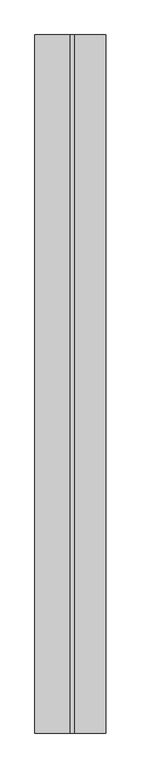
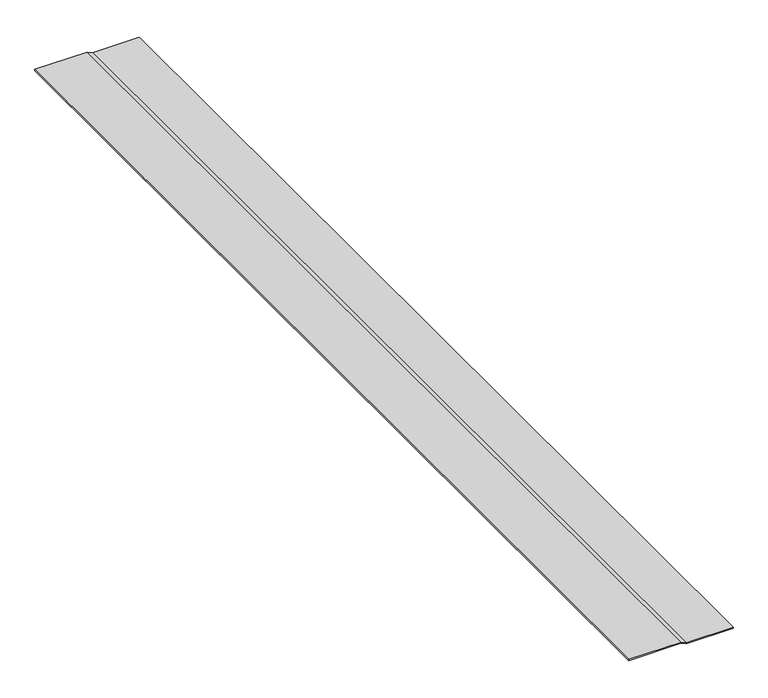
"""IFC4 building model written with IfcOpenShell, lengths in millimetres: proxy geometry, INTERPLY 4077 : INTERPLY 4077."""

from ifc_helpers import new_model, si_unit, frame, origin, place, context, project, spatial, polyline, outline, extrude, source, transform, mapped, element, save


def generic_models_f38cca31(model_context):
    return source(origin(), model_context, "Body", "SweptSolid", [
        extrude(outline(polyline([(40265.8733085, -2677.2016654), (40265.8733085, -2778.9380547), (40263.5642176, -2778.9380547), (40263.5642176, -2677.6931567), (40258.8529944, -2667.127576), (40258.8529944, -2575.8980157), (40261.1620854, -2575.8980157), (40261.1620854, -2666.6360847), (40265.8733085, -2677.2016654)])), frame((0.0, -1052.8906574, 0.0), z_axis=(0.0, 1.0, 0.0), x_axis=(0.0, 0.0, 1.0)), (0.0, 0.0, 1.0), 2000.25),
    ])


if __name__ == "__main__":
    model = new_model("IFC4")
    model_context = context("Model", 3, world=origin())
    ifc_project = project(units=[si_unit("LENGTHUNIT", "METRE", prefix="MILLI")], contexts=[model_context])
    site = spatial("IfcSite", under=ifc_project)
    building = spatial("IfcBuilding", under=site)
    placement = place(None, origin())
    generic_models_shape = generic_models_f38cca31(model_context)
    element("IfcBuildingElementProxy", 1, Name="INTERPLY 4077 : INTERPLY 4077", ObjectType="INTERPLY 4077 : INTERPLY 4077", at=placement, inside=building, context=model_context, shape_type="MappedRepresentation", body=[
        mapped(generic_models_shape, transform((0.0, 0.0, 0.0), x_axis=(1.0, 0.0, 0.0), y_axis=(0.0, 1.0, 0.0), z_axis=(0.0, 0.0, 1.0))),
    ])
    save(model, "model.ifc")

# Revit data of these elements
# Type "INTERPLY 4077 : INTERPLY 4077"
#   NameOverride = "INTERPLY"
# Element 1 (IfcBuildingElementProxy, "INTERPLY 4077 : INTERPLY 4077")
#   Materials on its faces: "INTERPLY REQUIRED FOR 15 & 20 YEARS SYSTEMS"
# Materials
#   "INTERPLY REQUIRED FOR 15 & 20 YEARS SYSTEMS": class "Unassigned", colour RGB 115 115 172, transparency 0
